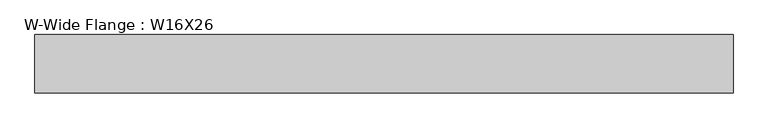
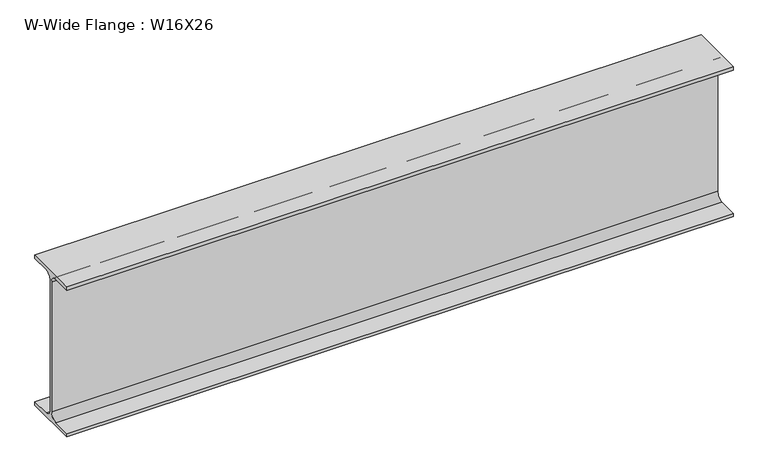
"""IFC4 building model written with IfcOpenShell, lengths in millimetres: beam geometry, W-Wide Flange : W16X26."""

import ifcopenshell
import ifcopenshell.guid

model = None  # the IFC model being written
_history = None  # IfcOwnerHistory: only IFC2X3 demands one
_inside = {}  # id of a spatial element -> (the spatial element, [elements in it])
_under = {}  # id of a project, library or spatial element -> (it, [spatial elements below it])
_declared = {}  # id of a project -> (the project, [libraries it declares])
_typed = {}  # id of a type object -> (the type object, [elements of that type])
_made_of = {}  # id of a material, layer set ... -> (it, [elements and type objects made of it])


def new_model(schema):
    """Start an empty IFC model of exactly this schema.

    Asked for "IFC4X3", IfcOpenShell would pick the latest addendum, in which some entities
    have other attributes; the version numbers below select the first issue.
    IFC2X3 requires an IfcOwnerHistory on every rooted entity: one is made here for all.
    """
    global model, _history
    if schema == "IFC4X3":
        model = ifcopenshell.file(schema_version=(4, 3, 0, 0))
    else:
        model = ifcopenshell.file(schema=schema)
    _inside.clear()
    _under.clear()
    _declared.clear()
    _typed.clear()
    _made_of.clear()
    _history = None
    if model.schema == "IFC2X3":
        org = make("IfcOrganization", Name="unknown")
        user = make(
            "IfcPersonAndOrganization",
            ThePerson=make("IfcPerson", FamilyName="unknown"),
            TheOrganization=org,
        )
        app = make(
            "IfcApplication",
            ApplicationDeveloper=org,
            Version="unknown",
            ApplicationFullName="unknown",
            ApplicationIdentifier="unknown",
        )
        _history = make(
            "IfcOwnerHistory",
            OwningUser=user,
            OwningApplication=app,
            ChangeAction="ADDED",
            CreationDate=0,
        )
    return model


def make(cls, **values):
    """One entity of the class cls with the attributes given. An attribute that is None is left unset."""
    return model.create_entity(
        cls, **{name: value for name, value in values.items() if value is not None}
    )


def rooted(cls, **values):
    """An entity with a GlobalId (a new one), such as an element, a storey or a relation."""
    return make(cls, GlobalId=ifcopenshell.guid.new(), OwnerHistory=_history, **values)


def si_unit(unit_type, name, prefix=None):
    """IfcSIUnit, for example si_unit("LENGTHUNIT", "METRE", prefix="MILLI")."""
    return make("IfcSIUnit", UnitType=unit_type, Prefix=prefix, Name=name)


def assignment(units):
    """IfcUnitAssignment: the units of a project."""
    return None if units is None else make("IfcUnitAssignment", Units=units)


def point(xyz):
    """IfcCartesianPoint."""
    return None if xyz is None else make("IfcCartesianPoint", Coordinates=xyz)


def direction(xyz):
    """IfcDirection."""
    return None if xyz is None else make("IfcDirection", DirectionRatios=xyz)


def frame(location, z_axis=None, x_axis=None):
    """IfcAxis2Placement3D, a coordinate frame: its origin and axes. An axis left out is left unset."""
    return make(
        "IfcAxis2Placement3D",
        Location=point(location),
        Axis=direction(z_axis),
        RefDirection=direction(x_axis),
    )


def frame_2d(location, x_axis=None):
    """IfcAxis2Placement2D, a coordinate frame in the plane: its origin and x axis."""
    return make(
        "IfcAxis2Placement2D", Location=point(location), RefDirection=direction(x_axis)
    )


def origin():
    """The frame at (0, 0, 0) with its axes left unset."""
    return frame((0.0, 0.0, 0.0))


def place(relative_to, where):
    """IfcLocalPlacement: puts the frame where relative to a parent placement (None: the world)."""
    return make(
        "IfcLocalPlacement", PlacementRelTo=relative_to, RelativePlacement=where
    )


def context(
    kind, dimensions, precision=None, world=None, true_north=None, identifier=None
):
    """IfcGeometricRepresentationContext, for example the 3D "Model" context."""
    return make(
        "IfcGeometricRepresentationContext",
        ContextIdentifier=identifier,
        ContextType=kind,
        CoordinateSpaceDimension=dimensions,
        Precision=precision,
        WorldCoordinateSystem=world,
        TrueNorth=true_north,
    )


def project(units=None, contexts=None):
    """IfcProject with its units and contexts."""
    return rooted(
        "IfcProject",
        Name="project",
        RepresentationContexts=contexts,
        UnitsInContext=assignment(units),
    )


def spatial(cls, under=None, at=None, **own):
    """A site, building, storey or space (cls), placed at a placement, below another one or the project."""
    s = rooted(cls, ObjectPlacement=at, **own)
    if under is not None:
        _under.setdefault(under.id(), (under, []))[1].append(s)
    return s


def polyline(points):
    """IfcPolyline through the points."""
    return make("IfcPolyline", Points=[point(p) for p in points])


def circle_curve(where, radius):
    """IfcCircle in the frame where."""
    return make("IfcCircle", Position=where, Radius=radius)


def trimmed(basis, trim1, trim2, sense, master):
    """IfcTrimmedCurve: the piece of a basis curve between two trims."""
    return make(
        "IfcTrimmedCurve",
        BasisCurve=basis,
        Trim1=trim1,
        Trim2=trim2,
        SenseAgreement=sense,
        MasterRepresentation=master,
    )


def segment(curve, same_sense, transition):
    """IfcCompositeCurveSegment."""
    return make(
        "IfcCompositeCurveSegment",
        Transition=transition,
        SameSense=same_sense,
        ParentCurve=curve,
    )


def composite_curve(segments, self_intersect=None):
    """IfcCompositeCurve: segments joined end to end."""
    return make("IfcCompositeCurve", Segments=segments, SelfIntersect=self_intersect)


def outline(outer, holes=None, kind="AREA"):
    """IfcArbitraryClosedProfileDef: a profile drawn as a closed curve; with holes, ...WithVoids."""
    if holes is None:
        return make("IfcArbitraryClosedProfileDef", ProfileType=kind, OuterCurve=outer)
    return make(
        "IfcArbitraryProfileDefWithVoids",
        ProfileType=kind,
        OuterCurve=outer,
        InnerCurves=holes,
    )


def extrude(swept, where, along, depth):
    """IfcExtrudedAreaSolid: the profile swept, set in the frame where, extruded along a direction by depth."""
    return make(
        "IfcExtrudedAreaSolid",
        SweptArea=swept,
        Position=where,
        ExtrudedDirection=direction(along),
        Depth=depth,
    )


def shape(context_of_items, identifier, shape_type, items):
    """IfcShapeRepresentation: the items that make up one representation, for example the "Body"."""
    return make(
        "IfcShapeRepresentation",
        ContextOfItems=context_of_items,
        RepresentationIdentifier=identifier,
        RepresentationType=shape_type,
        Items=items,
    )


def source(mapping_origin, context_of_items, identifier, shape_type, items):
    """IfcRepresentationMap: a shape defined once, which mapped items show again and again."""
    return make(
        "IfcRepresentationMap",
        MappingOrigin=mapping_origin,
        MappedRepresentation=shape(context_of_items, identifier, shape_type, items),
    )


def transform(
    local_origin,
    x_axis=None,
    y_axis=None,
    z_axis=None,
    scale=None,
    scale2=None,
    scale3=None,
    uniform=True,
):
    """IfcCartesianTransformationOperator3D, or its non-uniform kind. x_axis, y_axis, z_axis: its Axis1, 2, 3."""
    if uniform:
        return make(
            "IfcCartesianTransformationOperator3D",
            Axis1=direction(x_axis),
            Axis2=direction(y_axis),
            LocalOrigin=point(local_origin),
            Scale=scale,
            Axis3=direction(z_axis),
        )
    return make(
        "IfcCartesianTransformationOperator3DnonUniform",
        Axis1=direction(x_axis),
        Axis2=direction(y_axis),
        LocalOrigin=point(local_origin),
        Scale=scale,
        Axis3=direction(z_axis),
        Scale2=scale2,
        Scale3=scale3,
    )


def mapped(mapping_source, mapping_target):
    """IfcMappedItem: shows the shape of a source again, moved by a transform."""
    return make(
        "IfcMappedItem", MappingSource=mapping_source, MappingTarget=mapping_target
    )


def made_of(thing, what):
    """Note that an element or type object is made of a material, layer set ...; save() writes the relation."""
    if what is not None:
        _made_of.setdefault(what.id(), (what, []))[1].append(thing)
    return thing


def element(
    cls,
    number,
    at=None,
    inside=None,
    cuts=None,
    type_object=None,
    material=None,
    context=None,
    identifier="Body",
    shape_type=None,
    held_by="IfcProductDefinitionShape",
    body=None,
    shapes=None,
    **own,
):
    """One element of the class cls, such as IfcWall. Its Tag is "e" and its number.

    at: its placement. inside: the storey or other place that contains it. cuts: it is an
    opening in that element (IfcRelVoidsElement). A single representation is given by context,
    identifier, shape_type and body (its items); several are given by shapes. held_by: the class
    of the entity that holds the representations. save() writes the other relations.
    """
    e = rooted(cls, Tag="e%d" % number, ObjectPlacement=at, **own)
    if body is not None:
        shapes = [shape(context, identifier, shape_type, body)]
    if shapes is not None:
        e.Representation = make(held_by, Representations=shapes)
    if inside is not None:
        _inside.setdefault(inside.id(), (inside, []))[1].append(e)
    if cuts is not None:
        rooted(
            "IfcRelVoidsElement", RelatingBuildingElement=cuts, RelatedOpeningElement=e
        )
    if type_object is not None:
        _typed.setdefault(type_object.id(), (type_object, []))[1].append(e)
    return made_of(e, material)


def aggregate(whole, parts):
    """IfcRelAggregates: a whole, such as a stair, and the parts it consists of."""
    return rooted("IfcRelAggregates", RelatingObject=whole, RelatedObjects=parts)


def save(model, path):
    """Write the relations noted so far, then the file.

    IfcRelAggregates (storeys below a building ...), IfcRelContainedInSpatialStructure (elements
    in a storey), IfcRelDefinesByType, IfcRelAssociatesMaterial and IfcRelDeclares: one each for
    every whole, place, type object, material and project.
    """
    for whole, parts in _under.values():
        aggregate(whole, parts)
    for where, things in _inside.values():
        rooted(
            "IfcRelContainedInSpatialStructure",
            RelatedElements=things,
            RelatingStructure=where,
        )
    for kind, things in _typed.values():
        rooted("IfcRelDefinesByType", RelatedObjects=things, RelatingType=kind)
    for what, things in _made_of.values():
        rooted("IfcRelAssociatesMaterial", RelatedObjects=things, RelatingMaterial=what)
    for by, libraries in _declared.values():
        rooted("IfcRelDeclares", RelatingContext=by, RelatedDefinitions=libraries)
    model.write(path)


def w_wide_flange_w16x26_041745b3(model_context):
    return source(origin(), model_context, "Body", "SweptSolid", [
        extrude(outline(composite_curve([segment(polyline([(69.85, -190.627), (69.85, -199.39), (-69.85, -199.39), (-69.85, -190.627), (-21.3995, -190.627)]), True, "CONTINUOUS"), segment(trimmed(circle_curve(frame_2d((-21.3995, -172.4025)), 18.2245), [point((-21.3995, -190.627))], [point((-3.175, -172.4025))], True, "CARTESIAN"), True, "CONTINUOUS"), segment(polyline([(-3.175, -172.4025), (-3.175, 172.4025)]), True, "CONTINUOUS"), segment(trimmed(circle_curve(frame_2d((-21.3995, 172.4025)), 18.2245), [point((-3.175, 172.4025))], [point((-21.3995, 190.627))], True, "CARTESIAN"), True, "CONTINUOUS"), segment(polyline([(-21.3995, 190.627), (-69.85, 190.627), (-69.85, 199.39), (69.85, 199.39), (69.85, 190.627), (21.3995, 190.627)]), True, "CONTINUOUS"), segment(trimmed(circle_curve(frame_2d((21.3995, 172.4025)), 18.2245), [point((21.3995, 190.627))], [point((3.175, 172.4025))], True, "CARTESIAN"), True, "CONTINUOUS"), segment(polyline([(3.175, 172.4025), (3.175, -172.4025)]), True, "CONTINUOUS"), segment(trimmed(circle_curve(frame_2d((21.3995, -172.4025)), 18.2245), [point((3.175, -172.4025))], [point((21.3995, -190.627))], True, "CARTESIAN"), True, "CONTINUOUS"), segment(polyline([(21.3995, -190.627), (69.85, -190.627)]), True, "CONTINUOUS")], self_intersect=False)), frame((-842.7639083, 0.0, 0.0), z_axis=(1.0, 0.0, 0.0), x_axis=(0.0, 1.0, 0.0)), (0.0, 0.0, 1.0), 1674.6466767),
    ])


if __name__ == "__main__":
    model = new_model("IFC4")
    model_context = context("Model", 3, world=origin())
    ifc_project = project(units=[si_unit("LENGTHUNIT", "METRE", prefix="MILLI")], contexts=[model_context])
    site = spatial("IfcSite", under=ifc_project)
    building = spatial("IfcBuilding", under=site)
    placement = place(None, origin())
    w_wide_flange_w16x26_shape = w_wide_flange_w16x26_041745b3(model_context)
    element("IfcBeam", 1, ObjectType="W-Wide Flange : W16X26", at=placement, inside=building, context=model_context, shape_type="MappedRepresentation", body=[
        mapped(w_wide_flange_w16x26_shape, transform((0.0, 0.0, 0.0), x_axis=(1.0, 0.0, 0.0), y_axis=(0.0, 1.0, 0.0), z_axis=(0.0, 0.0, 1.0))),
    ])
    save(model, "model.ifc")

# Revit data of these elements
# Type "W-Wide Flange : W16X26"
#   Assembly Code = "B10"
#   W = 26
#   Length [instance default] = 5' - 0"
#   bf = 0' - 5 1/2"
#   d = 1' - 3.7"
#   k = 0' - 1 1/16"
#   k2 = 0' - 0.7175"
#   tf = 0' - 0.345"
#   tw = 0' - 0 1/4"
#   A = 0.0533333 SF
#   Structural Material [instance default] = Steel ASTM A992
# Element 1 (IfcBeam, "W-Wide Flange : W16X26")
#   Structural Material = Steel ASTM A36
#   Materials on its faces: "Steel ASTM A36"
# Materials
#   "Steel ASTM A992": class "Metal", colour RGB 199 199 199, transparency 0, Description = "Structural steel 50ksi", Cost = 0
#   "Steel ASTM A36": class "Metal", colour RGB 199 199 199, transparency 0, Description = "Structural steel, ASTM A36 Grade B, mill finish", Cost = 0
